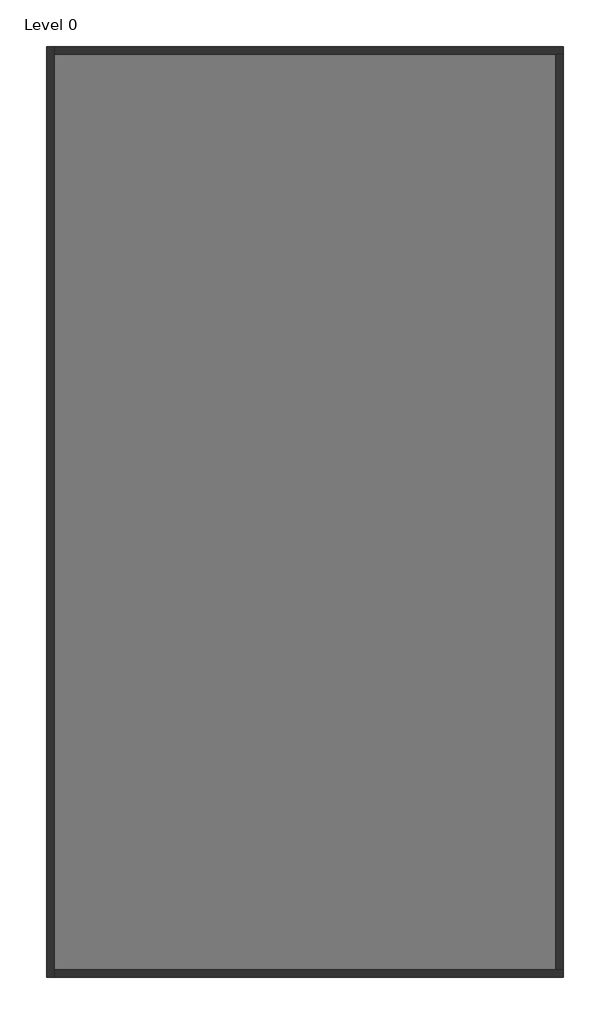
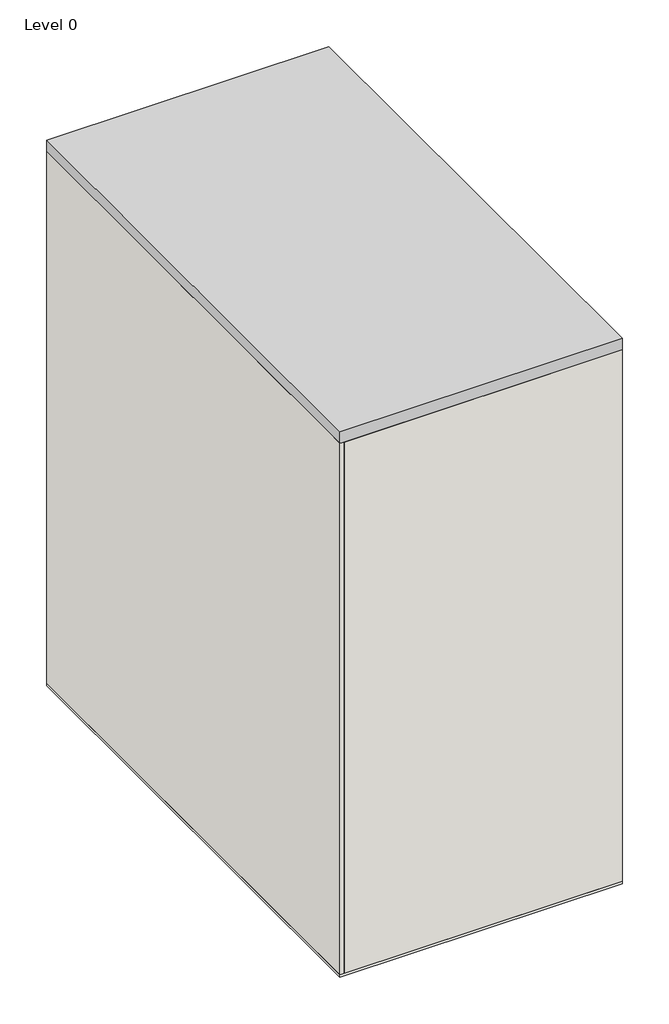
# One storey: 4 walls, 1 proxy, 1 slab.
"""IFC4 building model written with IfcOpenShell, lengths in millimetres."""

from ifc_helpers import new_model, si_unit, frame, origin, origin_with_axes, place, context, project, spatial, polyline, outline, extrude, faceted_brep, element, save

model = new_model("IFC4")

# Units and contexts
model_context = context("Model", 3, world=origin())
ifc_project = project(units=[si_unit("LENGTHUNIT", "METRE", prefix="MILLI")], contexts=[model_context])

# Site, building, storey
site = spatial("IfcSite", under=ifc_project)
building = spatial("IfcBuilding", under=site)
storey = spatial("IfcBuildingStorey", under=building, Name="Level 0", Elevation=100.0)

# Proxy
placement = place(None, origin())
element("IfcBuildingElementProxy", 1, Name="LowUrbanDensityBuilding : LowUrbanDensityBuilding", ObjectType="LowUrbanDensityBuilding : LowUrbanDensityBuilding", at=placement, inside=storey, context=model_context, shape_type="SweptSolid", body=[
    extrude(outline(polyline([(7325.2659446, 3676.2074539), (7325.2659446, -14323.7925461), (-2674.7340554, -14323.7925461), (-2674.7340554, 3676.2074539), (7325.2659446, 3676.2074539)])), origin_with_axes(), (0.0, 0.0, 1.0), 20445.0),
])

# Slab
element("IfcSlab", 2, ObjectType="Floor-Concrete_100Con", at=placement, inside=storey, context=model_context, shape_type="SweptSolid", body=[
    extrude(outline(polyline([(7325.2659446, 3676.2074539), (7325.2659446, -14323.7925461), (-2674.7340554, -14323.7925461), (-2674.7340554, 3676.2074539), (7325.2659446, 3676.2074539)])), origin_with_axes(), (0.0, 0.0, 1.0), 100.0),
])

# Walls
element("IfcWall", 3, ObjectType="Wall-Ext_25Rdr-100Blk-19P", at=placement, inside=storey, context=model_context, shape_type="Brep", body=[
    faceted_brep([(-2674.7340554, 3676.2074539, 100.0), (-2674.7340554, -14323.7925461, 100.0), (-2674.7340554, -14323.7925461, 20000.0), (-2674.7340554, 3676.2074539, 20000.0), (-2530.4340554, 3676.2074539, 100.0), (-2530.4340554, 3676.2074539, 20000.0), (-2530.4340554, 3531.9074539, 20000.0), (-2530.4340554, -14179.4925461, 20000.0), (-2530.4340554, -14323.7925461, 20000.0), (-2530.4340554, -14323.7925461, 100.0), (-2530.4340554, -14179.4925461, 100.0), (-2530.4340554, 3531.9074539, 100.0)], [[[0, 1, 2, 3]], [[4, 5, 6, 7, 8, 9, 10, 11]], [[1, 0, 4, 11, 10, 9]], [[3, 2, 8, 7, 6, 5]], [[2, 1, 9, 8]], [[0, 3, 5, 4]]]),
])
element("IfcWall", 4, ObjectType="Wall-Ext_25Rdr-100Blk-19P", at=placement, inside=storey, context=model_context, shape_type="Brep", body=[
    faceted_brep([(-2530.4340554, -14323.7925461, 100.0), (7325.2659446, -14323.7925461, 100.0), (7325.2659446, -14323.7925461, 20000.0), (-2530.4340554, -14323.7925461, 20000.0), (-2530.4340554, -14179.4925461, 100.0), (-2530.4340554, -14179.4925461, 20000.0), (7180.9659446, -14179.4925461, 20000.0), (7325.2659446, -14179.4925461, 20000.0), (7325.2659446, -14179.4925461, 100.0), (7180.9659446, -14179.4925461, 100.0)], [[[0, 1, 2, 3]], [[4, 5, 6, 7, 8, 9]], [[1, 0, 4, 9, 8]], [[3, 2, 7, 6, 5]], [[0, 3, 5, 4]], [[2, 1, 8, 7]]]),
])
element("IfcWall", 5, ObjectType="Wall-Ext_25Rdr-100Blk-19P", at=placement, inside=storey, context=model_context, shape_type="Brep", body=[
    faceted_brep([(7325.2659446, 3676.2074539, 100.0), (-2530.4340554, 3676.2074539, 100.0), (-2530.4340554, 3676.2074539, 20000.0), (7325.2659446, 3676.2074539, 20000.0), (7325.2659446, 3531.9074539, 100.0), (7325.2659446, 3531.9074539, 20000.0), (7180.9659446, 3531.9074539, 20000.0), (-2530.4340554, 3531.9074539, 20000.0), (-2530.4340554, 3531.9074539, 100.0), (7180.9659446, 3531.9074539, 100.0)], [[[0, 1, 2, 3]], [[4, 5, 6, 7, 8, 9]], [[1, 0, 4, 9, 8]], [[3, 2, 7, 6, 5]], [[2, 1, 8, 7]], [[0, 3, 5, 4]]]),
])
element("IfcWall", 6, ObjectType="Wall-Ext_25Rdr-100Blk-19P", at=placement, inside=storey, context=model_context, shape_type="SweptSolid", body=[
    extrude(outline(polyline([(7325.2659446, 3531.9074539), (7325.2659446, -14179.4925461), (7180.9659446, -14179.4925461), (7180.9659446, 3531.9074539), (7325.2659446, 3531.9074539)])), frame((0.0, 0.0, 100.0), z_axis=(0.0, 0.0, 1.0), x_axis=(1.0, 0.0, 0.0)), (0.0, 0.0, 1.0), 19900.0),
])

save(model, "model.ifc")

# Revit data of these elements
# Project information
#   Project Issue Date = "Issue Date"
#   Project Status = "Project Status"
#   Client Name = "Owner"
#   Project Address = "Enter address here"
#   Project Name = "Project Name"
#   Project Number = "Project Number"
# Type "Floor-Concrete_100Con"
#   Keynote = "E60/130"
#   Function = 0
#   Layers, outside or top first: 100 mm "Concrete" (function 1)
# Type "Wall-Ext_25Rdr-100Blk-19P"
#   Keynote = "F10"
#   Layers, outside or top first: 25.3 mm "Render, Beige, Smooth" (function 5); 100 mm "Concrete Masonry Units _Low Density" (function 1); 19 mm "Plaster" (function 5)
# Element 1 (IfcBuildingElementProxy, "LowUrbanDensityBuilding : LowUrbanDensityBuilding")
#   Phase Created = New Construction
#   Materials on its faces: "Default Form"
# Element 2 (IfcSlab, "Floor-Concrete_100Con")
#   Height Offset From Level = 0 mm
#   Phase Created = New Construction
#   Materials on its faces: "Concrete"
# Element 3 (IfcWall, "Wall-Ext_25Rdr-100Blk-19P")
#   Top Offset = 0 mm
#   Base Offset = 0 mm
#   wall height = 19900 mm
#   Phase Created = New Construction
#   Base Constraint = Level 0
#   Top Constraint = Level 5
#   Materials on its faces: "Render, Beige, Smooth", "Default Wall", "Plaster"
# Elements 4, 5, 6 (IfcWall, "Wall-Ext_25Rdr-100Blk-19P")
#   Top Offset = 0 mm
#   Base Offset = 0 mm
#   wall height = 19900 mm
#   Phase Created = New Construction
#   Base Constraint = Level 0
#   Top Constraint = Level 5
#   Materials on its faces: "Default Wall", "Render, Beige, Smooth", "Plaster"
# Materials
#   "Concrete": class "Concrete", colour RGB 120 120 120, transparency 0, Description = "Portland Cement Concrete", Cost = 0
#   "Render, Beige, Smooth": class "Generic", colour RGB 213 198 180, transparency 0, Description = "physical material", Cost = 0
#   "Concrete Masonry Units _Low Density": class "Masonry", colour RGB 181 181 181, transparency 0, Description = "Concrete masonry units", Cost = 0
#   "Plaster": class "Generic", colour RGB 249 249 249, transparency 0, Description = "Plaster", Cost = 0
#   "Default Form": class "Generic", colour RGB 185 189 196, transparency 0.5, Cost = 0
#   "Default Wall": class "Miscellaneous", colour RGB 128 128 128, transparency 0, Comments = "Rendering appearance not upgraded Rendering appearance not upgraded ", Cost = 0
